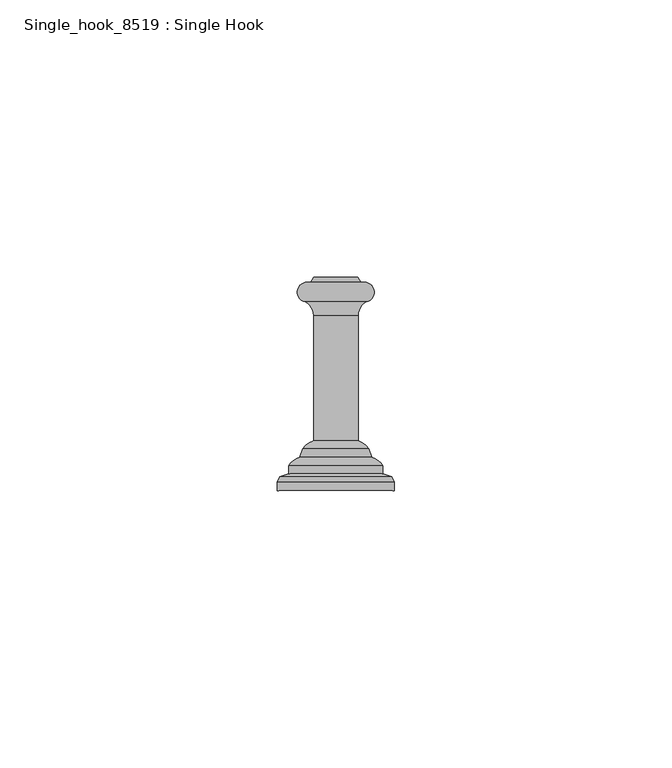
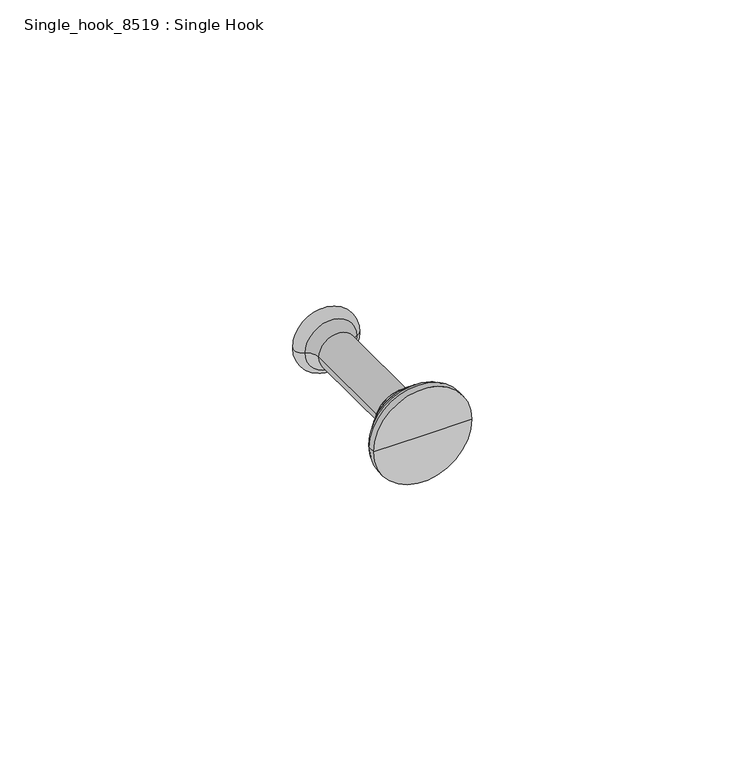
"""IFC4 building model written with IfcOpenShell, lengths in millimetres: proxy geometry, Single_hook_8519 : Single Hook."""

from ifc_helpers import new_model, si_unit, point, frame, origin, place, context, project, spatial, polyline, circle_curve, ellipse_curve, trimmed, source, transform, mapped, element, save
from ifc_brep_helpers import plane_surface, cylinder_surface, revolved_surface, advanced_brep


def single_hook_8519_single_hook_65f89b15(model_context):
    return source(origin(), model_context, "Body", "AdvancedBrep", [
        advanced_brep(
        [(120.4999999, 108.9374993, 0.0), (129.5000001, 108.9374993, 0.0), (130.5000004, 108.9374993, 0.0), (119.4999996, 108.9374993, 0.0), (121.0086329, 109.8184776, 0.0), (128.9913671, 109.8184776, 0.0), (125.0, 109.8184776, 0.0), (114.5000005, 71.4375, 0.0), (135.4999995, 71.4375, 0.0), (125.0, 71.4375, 0.0), (114.5000005, 72.9561938, 0.0), (135.4999995, 72.9561938, 0.0), (114.8940547, 73.8845273, 0.0), (135.1059453, 73.8845273, 0.0), (116.4999999, 74.4374986, 0.0), (133.5000001, 74.4374986, 0.0), (116.4999999, 75.9034491, 0.0), (133.5000001, 75.9034491, 0.0), (118.489313, 77.4576708, 0.0), (131.510687, 77.4576708, 0.0), (119.0341392, 78.9545686, 0.0), (130.9658608, 78.9545686, 0.0), (120.9909169, 80.4291064, 0.0), (129.0090831, 80.4291064, 0.0), (120.9909169, 102.9266117, 0.0), (129.0090831, 102.9266117, 0.0), (119.4999996, 105.4374993, 0.0), (130.5000004, 105.4374993, 0.0)],
        [
            (0, 1, circle_curve(frame((125.0, 108.9374993, 0.0), z_axis=(0.0, -1.0, 0.0), x_axis=(1.0, 0.0, 0.0)), 4.5000001)),
            (1, 2),
            (2, 3, circle_curve(frame((125.0, 108.9374993, 0.0), z_axis=(0.0, 1.0, 0.0), x_axis=(1.0, 0.0, 0.0)), 5.5000004)),
            (3, 0),
            (1, 0, circle_curve(frame((125.0, 108.9374993, 0.0), z_axis=(0.0, -1.0, 0.0), x_axis=(1.0, 0.0, 0.0)), 4.5000001)),
            (3, 2, circle_curve(frame((125.0, 108.9374993, 0.0), z_axis=(0.0, 1.0, 0.0), x_axis=(1.0, 0.0, 0.0)), 5.5000004)),
            (4, 5, circle_curve(frame((125.0, 109.8184776, 0.0), z_axis=(0.0, -1.0, 0.0), x_axis=(1.0, 0.0, 0.0)), 3.9913671)),
            (5, 1),
            (0, 4),
            (5, 4, circle_curve(frame((125.0, 109.8184776, 0.0), z_axis=(0.0, -1.0, 0.0), x_axis=(1.0, 0.0, 0.0)), 3.9913671)),
            (6, 5),
            (4, 6),
            (7, 8, circle_curve(frame((125.0, 71.4375, 0.0), z_axis=(0.0, -1.0, 0.0), x_axis=(1.0, 0.0, 0.0)), 10.4999995)),
            (8, 9),
            (9, 7),
            (8, 7, circle_curve(frame((125.0, 71.4375, 0.0), z_axis=(0.0, -1.0, 0.0), x_axis=(1.0, 0.0, 0.0)), 10.4999995)),
            (10, 11, circle_curve(frame((125.0, 72.9561938, 0.0), z_axis=(0.0, -1.0, 0.0), x_axis=(1.0, 0.0, 0.0)), 10.4999995)),
            (11, 8),
            (7, 10),
            (11, 10, circle_curve(frame((125.0, 72.9561938, 0.0), z_axis=(0.0, -1.0, 0.0), x_axis=(1.0, 0.0, 0.0)), 10.4999995)),
            (12, 13, circle_curve(frame((125.0, 73.8845273, 0.0), z_axis=(0.0, -1.0, 0.0), x_axis=(1.0, 0.0, 0.0)), 10.1059453)),
            (13, 11),
            (10, 12),
            (13, 12, circle_curve(frame((125.0, 73.8845273, 0.0), z_axis=(0.0, -1.0, 0.0), x_axis=(1.0, 0.0, 0.0)), 10.1059453)),
            (14, 15, circle_curve(frame((125.0, 74.4374986, 0.0), z_axis=(0.0, -1.0, 0.0), x_axis=(1.0, 0.0, 0.0)), 8.5000001)),
            (15, 13),
            (12, 14),
            (15, 14, circle_curve(frame((125.0, 74.4374986, 0.0), z_axis=(0.0, -1.0, 0.0), x_axis=(1.0, 0.0, 0.0)), 8.5000001)),
            (16, 17, circle_curve(frame((125.0, 75.9034491, 0.0), z_axis=(0.0, -1.0, 0.0), x_axis=(1.0, 0.0, 0.0)), 8.5000001)),
            (17, 15),
            (14, 16),
            (17, 16, circle_curve(frame((125.0, 75.9034491, 0.0), z_axis=(0.0, -1.0, 0.0), x_axis=(1.0, 0.0, 0.0)), 8.5000001)),
            (18, 19, circle_curve(frame((125.0, 77.4576708, 0.0), z_axis=(0.0, -1.0, 0.0), x_axis=(1.0, 0.0, 0.0)), 6.510687)),
            (19, 17, circle_curve(frame((130.1450927, 73.6595765, 0.0), z_axis=(0.0, 0.0, -1.0), x_axis=(1.0, 0.0, 0.0)), 4.0361328)),
            (16, 18, circle_curve(frame((119.8549073, 73.6595765, 0.0), z_axis=(0.0, 0.0, -1.0), x_axis=(-1.0, 0.0, 0.0)), 4.0361328)),
            (19, 18, circle_curve(frame((125.0, 77.4576708, 0.0), z_axis=(0.0, -1.0, 0.0), x_axis=(1.0, 0.0, 0.0)), 6.510687)),
            (20, 21, circle_curve(frame((125.0, 78.9545686, 0.0), z_axis=(0.0, -1.0, 0.0), x_axis=(1.0, 0.0, 0.0)), 5.9658608)),
            (21, 19),
            (18, 20),
            (21, 20, circle_curve(frame((125.0, 78.9545686, 0.0), z_axis=(0.0, -1.0, 0.0), x_axis=(1.0, 0.0, 0.0)), 5.9658608)),
            (22, 23, circle_curve(frame((125.0, 80.4291064, 0.0), z_axis=(0.0, -1.0, 0.0), x_axis=(1.0, 0.0, 0.0)), 4.0090831)),
            (23, 21, circle_curve(frame((127.5885586, 76.5083721, 0.0), z_axis=(0.0, 0.0, -1.0), x_axis=(1.0, 0.0, 0.0)), 4.1701376)),
            (20, 22, circle_curve(frame((122.4114414, 76.5083721, 0.0), z_axis=(0.0, 0.0, -1.0), x_axis=(-1.0, 0.0, 0.0)), 4.1701376)),
            (23, 22, circle_curve(frame((125.0, 80.4291064, 0.0), z_axis=(0.0, -1.0, 0.0), x_axis=(1.0, 0.0, 0.0)), 4.0090831)),
            (24, 25, circle_curve(frame((125.0, 102.9266117, 0.0), z_axis=(0.0, -1.0, 0.0), x_axis=(1.0, 0.0, 0.0)), 4.0090831)),
            (25, 23),
            (22, 24),
            (25, 24, circle_curve(frame((125.0, 102.9266117, 0.0), z_axis=(0.0, -1.0, 0.0), x_axis=(1.0, 0.0, 0.0)), 4.0090831)),
            (26, 27, circle_curve(frame((125.0, 105.4374993, 0.0), z_axis=(0.0, -1.0, 0.0), x_axis=(1.0, 0.0, 0.0)), 5.5000004)),
            (27, 25, circle_curve(frame((131.8688631, 102.9266117, 0.0), z_axis=(0.0, 0.0, 1.0), x_axis=(1.0, 0.0, 0.0)), 2.85978)),
            (24, 26, circle_curve(frame((118.1311369, 102.9266117, 0.0), z_axis=(0.0, 0.0, 1.0), x_axis=(-1.0, 0.0, 0.0)), 2.85978)),
            (27, 26, circle_curve(frame((125.0, 105.4374993, 0.0), z_axis=(0.0, -1.0, 0.0), x_axis=(1.0, 0.0, 0.0)), 5.5000004)),
            (2, 27, circle_curve(frame((130.125001, 107.1874993, 0.0), z_axis=(0.0, 0.0, -1.0), x_axis=(1.0, 0.0, 0.0)), 1.7897275)),
            (26, 3, circle_curve(frame((119.874999, 107.1874993, 0.0), z_axis=(0.0, 0.0, -1.0), x_axis=(-1.0, 0.0, 0.0)), 1.7897275)),
        ],
        [
            plane_surface(frame((125.0, 108.9374993, 0.0), z_axis=(0.0, 1.0, 0.0), x_axis=(1.0, 0.0, 0.0))),
            revolved_surface(polyline([(129.5000001, 108.9374993, 0.0), (128.9913671, 109.8184776, 0.0)]), (125.0, 127.3855881, 0.0), (0.0, 1.0, 0.0)),
            plane_surface(frame((125.0, 109.8184776, 0.0), z_axis=(0.0, 1.0, 0.0), x_axis=(1.0, 0.0, 0.0))),
            plane_surface(frame((125.0, 71.4375, 0.0), z_axis=(0.0, -1.0, 0.0), x_axis=(1.0, 0.0, 0.0))),
            cylinder_surface(frame((125.0, 127.3855881, 0.0), z_axis=(0.0, 1.0, 0.0), x_axis=(1.0, 0.0, 0.0)), 10.4999995),
            revolved_surface(polyline([(135.4999995, 72.9561938, 0.0), (135.1059453, 73.8845273, 0.0)]), (125.0, 127.3855881, 0.0), (0.0, 1.0, 0.0)),
            revolved_surface(polyline([(135.1059453, 73.8845273, 0.0), (133.5000001, 74.4374986, 0.0)]), (125.0, 127.3855881, 0.0), (0.0, 1.0, 0.0)),
            cylinder_surface(frame((125.0, 127.3855881, 0.0), z_axis=(0.0, 1.0, 0.0), x_axis=(1.0, 0.0, 0.0)), 8.5000001),
            revolved_surface(trimmed(ellipse_curve(frame((130.1450927, 73.6595765, 0.0), z_axis=(0.0, 0.0, 1.0), x_axis=(1.0, 0.0, 0.0)), 4.0361328, 4.0361328), [point((133.5000001, 75.9034491, 0.0))], [point((131.510687, 77.4576708, 0.0))], True, "CARTESIAN"), (125.0, 127.3855881, 0.0), (0.0, 1.0, 0.0)),
            revolved_surface(polyline([(131.510687, 77.4576708, 0.0), (130.9658608, 78.9545686, 0.0)]), (125.0, 127.3855881, 0.0), (0.0, 1.0, 0.0)),
            revolved_surface(trimmed(ellipse_curve(frame((127.5885586, 76.5083721, 0.0), z_axis=(0.0, 0.0, 1.0), x_axis=(1.0, 0.0, 0.0)), 4.1701376, 4.1701376), [point((130.9658608, 78.9545686, 0.0))], [point((129.0090831, 80.4291064, 0.0))], True, "CARTESIAN"), (125.0, 127.3855881, 0.0), (0.0, 1.0, 0.0)),
            cylinder_surface(frame((125.0, 127.3855881, 0.0), z_axis=(0.0, 1.0, 0.0), x_axis=(1.0, 0.0, 0.0)), 4.0090831),
            revolved_surface(trimmed(ellipse_curve(frame((131.8688631, 102.9266117, 0.0), z_axis=(0.0, 0.0, -1.0), x_axis=(1.0, 0.0, 0.0)), 2.85978, 2.85978), [point((129.0090831, 102.9266117, 0.0))], [point((130.5000004, 105.4374993, 0.0))], True, "CARTESIAN"), (125.0, 127.3855881, 0.0), (0.0, 1.0, 0.0)),
            revolved_surface(trimmed(ellipse_curve(frame((130.125001, 107.1874993, 0.0), z_axis=(0.0, 0.0, 1.0), x_axis=(1.0, 0.0, 0.0)), 1.7897275, 1.7897275), [point((130.5000004, 105.4374993, 0.0))], [point((130.5000004, 108.9374993, 0.0))], True, "CARTESIAN"), (125.0, 127.3855881, 0.0), (0.0, 1.0, 0.0)),
        ],
        [
            (0, [[1, 2, 3, 4]]),
            (0, [[5, -4, 6, -2]]),
            (1, [[7, 8, -1, 9]]),
            (1, [[10, -9, -5, -8]]),
            (2, [[11, -7, 12]]),
            (2, [[-12, -10, -11]]),
            (3, [[13, 14, 15]]),
            (3, [[16, -15, -14]]),
            (4, [[17, 18, -13, 19]]),
            (4, [[20, -19, -16, -18]]),
            (5, [[21, 22, -17, 23]]),
            (5, [[24, -23, -20, -22]]),
            (6, [[25, 26, -21, 27]]),
            (6, [[28, -27, -24, -26]]),
            (7, [[29, 30, -25, 31]]),
            (7, [[32, -31, -28, -30]]),
            (8, [[33, 34, -29, 35]]),
            (8, [[36, -35, -32, -34]]),
            (9, [[37, 38, -33, 39]]),
            (9, [[40, -39, -36, -38]]),
            (10, [[41, 42, -37, 43]]),
            (10, [[44, -43, -40, -42]]),
            (11, [[45, 46, -41, 47]]),
            (11, [[48, -47, -44, -46]]),
            (12, [[49, 50, -45, 51]]),
            (12, [[52, -51, -48, -50]]),
            (13, [[-3, 53, -49, 54]]),
            (13, [[-6, -54, -52, -53]]),
        ],
    ),
    ])


if __name__ == "__main__":
    model = new_model("IFC4")
    model_context = context("Model", 3, world=origin())
    ifc_project = project(units=[si_unit("LENGTHUNIT", "METRE", prefix="MILLI")], contexts=[model_context])
    site = spatial("IfcSite", under=ifc_project)
    building = spatial("IfcBuilding", under=site)
    placement = place(None, origin())
    single_hook_8519_single_hook_shape = single_hook_8519_single_hook_65f89b15(model_context)
    element("IfcBuildingElementProxy", 1, Name="Single_hook_8519 : Single Hook", ObjectType="Single_hook_8519 : Single Hook", at=placement, inside=building, context=model_context, shape_type="MappedRepresentation", body=[
        mapped(single_hook_8519_single_hook_shape, transform((0.0, 0.0, 0.0), x_axis=(1.0, 0.0, 0.0), y_axis=(0.0, 1.0, 0.0), z_axis=(0.0, 0.0, 1.0))),
    ])
    save(model, "model.ifc")

# Revit data of these elements
# Type "Single_hook_8519 : Single Hook"
#   URL = "http://www.hansgrohe.co.uk/uk_en/110585_32313931335F32355F3632303236.htm"
#   Model = "Montreux 42137830"
#   Manufacturer = "Axor"
#   Keynote = "10800.A9"
#   Description = "Polished Nickel"
#   Wall Center Offset [instance default] = 0' - 2.95276"
#   Assembly Code = ""
# Element 1 (IfcBuildingElementProxy, "Single_hook_8519 : Single Hook")
#   Wall Center Offset = 0' - 0"
#   Materials on its faces: "Chrome"
# Materials
#   "Chrome": class "Metal", colour RGB 152 152 152, transparency 0
